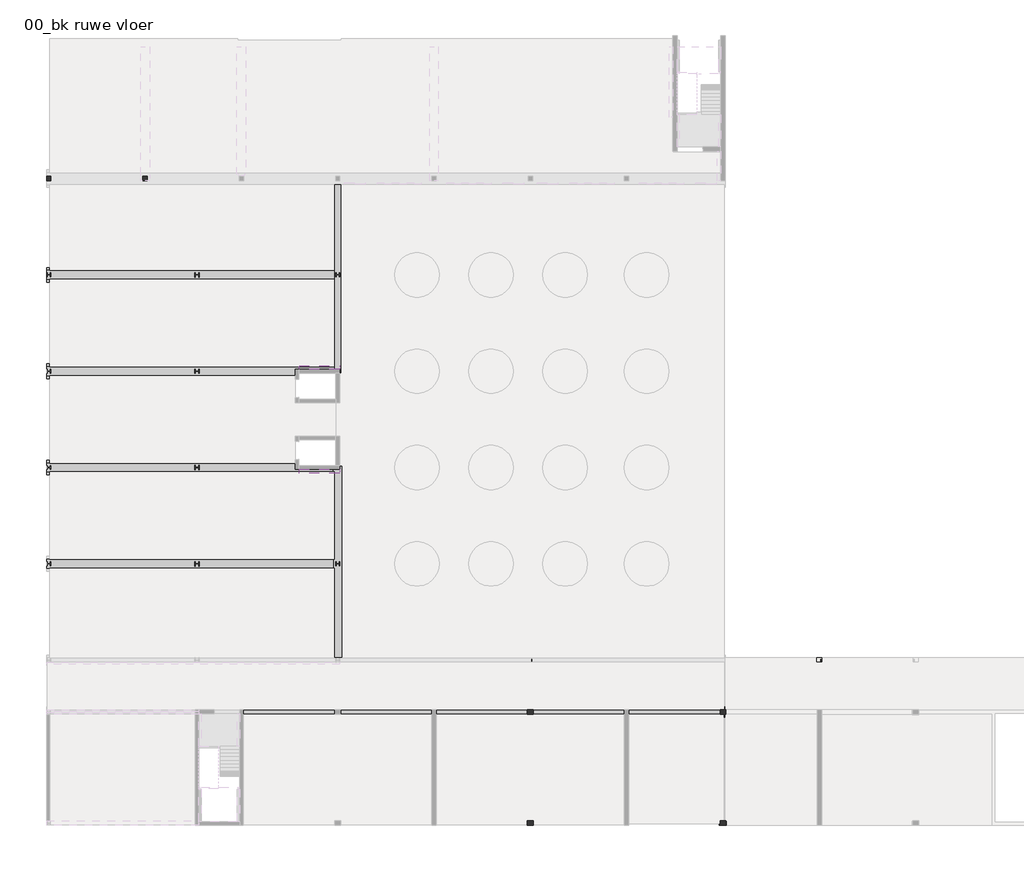
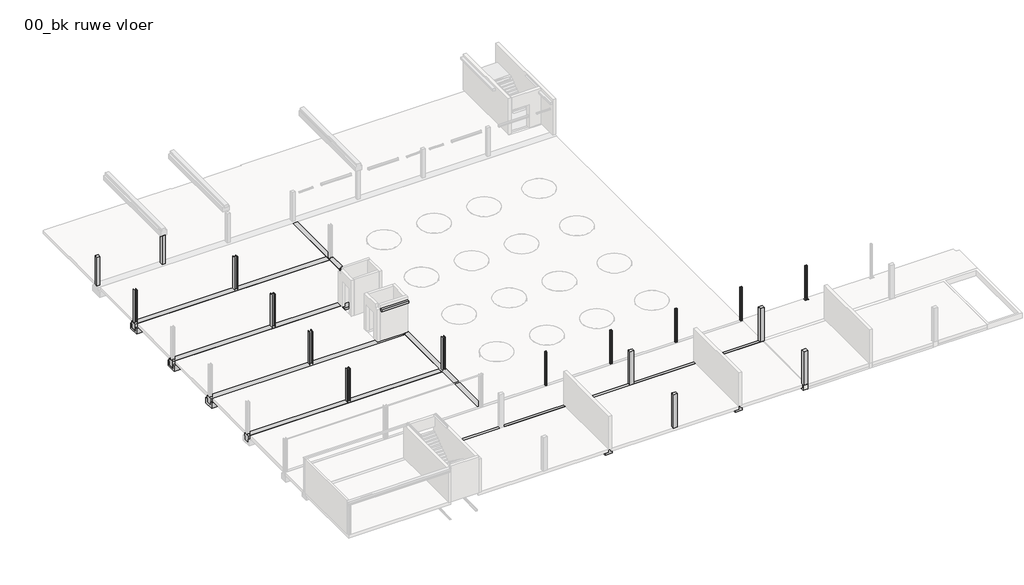
# One storey, part 5 of 6: 17 columns, 14 beams, 2 slabs.
# Revit data of these elements (continued)
# Type "NLRS_28_SF_LIB_balk dubbele sponning beton ihwg-CWV-MMBC-SRP_gen_rsf : balk beton ihwg_gen__bxh 900x900 met inkassing bxh 200x320" (continued)
#   RSF_C_breedte_inkassing_rechts = 200 mm
#   RSF_C_breedte_inkassing_links = 200 mm
#   NLRS_C_lengte [instance default] = 3000 mm
#   NLRS_C_hoogte = 900 mm
#   NLRS_C_breedte = 900 mm
#   Length [instance default] = 3000 mm
#   Structural Material = NLRS_f2_beton ihwg_gen_rsf
#   Model = ""
# Type "NLRS_22_SF_LIB_oplegnok beton prefab framing-CWV-MMBPC-SRP_gen_rsf : oplegnok beton prefab_gen__bxh 250x250/220"
#   Export Type to IFC As = "IfcWallType"
#   Type IfcGUID = "3EzArCxHzFqA2seU7O0xFZ"
#   Type Comments = "oplegnok"
#   Model = "LOD300"
#   Description = "oplegnok beton prefab 250x250/220"
#   Assembly Code = "22.11"
#   NLRS_C_hoogte_01 = 220 mm
#   NLRS_C_hoogte = 250 mm
#   NLRS_C_breedte = 250 mm
#   Lossing = 30 mm
#   Length [instance default] = 3000 mm
#   Structural Material = NLRS_f2_beton prefab_gen_rsf
# Type "NLRS_28_SCO_TLB_stalen kolom HEA-BCPG-MMBS-SRP_gen_rsf : stalen kolom_gen__HEA 260"
#   Type IFC Predefined Type = "COLUMN"
#   Export Type to IFC As = "IfcColumnType"
#   Type IfcGUID = "2$hNzCXOT3YR8V$0CfyzGd"
#   Type Comments = "HEA260"
#   Model = " "
#   Manufacturer = " "
#   Description = "stalen kolom HEA260"
#   Assembly Code = "28.11"
#   vz = 125 mm
#   vy = 130 mm
#   vpz = 125 mm
#   vpy = 130 mm
#   tw = 7.5 mm
#   tf = 12.5 mm
#   ra = 24 mm
#   d = 250 mm
#   bf = 260 mm
#   NLRS_C_lengte [instance default] = 2743.2 mm
#   Structural Material = NLRS_h2_staal_gen_rsf
#   Keynote = ""
# Type "NLRS_28_SCO_TLB_vierkante kolom beton prefab-BCPG-MMBPC-SRP_gen_rsf : kolom vierkant beton prefab_gen__bxh 300x300"
#   Type IFC Predefined Type = "COLUMN"
#   Export Type to IFC As = "IfcColumnType"
#   Type IfcGUID = "2bNskL0kfByRmbY5G6If0x"
#   Type Comments = "300x300"
#   Model = "LOD300"
#   Description = "prefab betonkolom 300x300"
#   Assembly Code = "28.11"
#   NLRS_C_lengte [instance default] = 2700 mm
#   NLRS_C_hoogte = 300 mm
#   NLRS_C_breedte = 300 mm
#   Structural Material = NLRS_f2_beton prefab_gen_rsf
# Type "NLRS_28_SCO_TLB_stalen kolom HEB-BCPG-MMBS-SRP_gen_rsf : stalen kolom_gen__HEB 300"
#   Type IFC Predefined Type = "COLUMN"
#   Export Type to IFC As = "IfcColumnType"
#   Type IfcGUID = "3C_b5Xdrv818Ti1jf59K4n"
#   Type Comments = "HEB300"
#   Model = " "
#   Manufacturer = " "
#   Description = "stalen kolom HEB300"
#   Assembly Code = "28.11"
#   vz = 150 mm
#   vy = 150 mm
#   vpz = 150 mm
#   vpy = 150 mm
#   tw = 11 mm
#   tf = 19 mm
#   ra = 27 mm
#   d = 300 mm
#   bf = 300 mm
#   NLRS_C_lengte [instance default] = 2743.2 mm
#   Structural Material = NLRS_h2_staal_gen_rsf
#   Keynote = ""
# Type "NLRS_28_SCO_TLB_vierkante kolom beton ihwg-BCPG-MMBC-SRP_gen_rsf : vierkante kolom beton ihwg_gen__bxh 400x300"
#   Type IFC Predefined Type = "COLUMN"
#   Export Type to IFC As = "IfcColumnType"
#   Type IfcGUID = "2lw04Qbvr9TgC3fLWwYn2N"
#   Type Comments = "400x300"
#   Model = "LOD300"
#   Description = "betonkolom ihwg 400x300"
#   Assembly Code = "28.11"
#   NLRS_C_lengte [instance default] = 2700 mm
#   NLRS_C_hoogte = 300 mm
#   NLRS_C_breedte = 400 mm
#   Structural Material = NLRS_f2_beton ihwg_gen_rsf
# Type "NLRS_28_SCO_TLB_stalen kolom buisprofiel koudgevormd vierkant-BCPG-MMBS-SRP_gen_rsf : stalen kolom buisprofiel koudgevormd vierkant RHSC_gen__160x160x8"
#   Type IFC Predefined Type = "COLUMN"
#   Export Type to IFC As = "IfcColumnType"
#   Type IfcGUID = "2$hNzCXOT3YR8V$0Cfyzxk"
#   Type Comments = "K160x160x8"
#   Model = " "
#   Manufacturer = " "
#   Description = "stalen kolom K160x160x8"
#   Assembly Code = "28.11"
#   vz = 80 mm
#   vy = 80 mm
#   vpz = 80 mm
#   vpy = 80 mm
#   tw = 8 mm
#   tf = 8 mm
#   ri = 20 mm
#   ra = 12 mm
#   d = 160 mm
#   bf = 160 mm
#   NLRS_C_lengte [instance default] = 2743.2 mm
#   Structural Material = NLRS_h2_staal_gen_rsf
#   Keynote = ""
# Type "NLRS_16_SFO_WPB_stiep rechthoek beton ihwg-AV-MMBC_gen_rsf : stiep beton ihwg_gen__bxl 300x400"
#   Export Type to IFC As = "IfcFootingType"
#   Type IfcGUID = "3aMdMHoe12P9KDGPyaIeli"
#   Type Comments = "stiep 300x400"
#   Description = "stiep 300x400"
#   Assembly Code = "16.13"
#   Width = 300 mm
#   NLRS_C_lengte = 400 mm
#   NLRS_C_hoogte [instance default] = 600 mm
#   NLRS_C_breedte = 300 mm
#   Length = 400 mm
#   Structural Material = NLRS_f2_beton ihwg_gen_rsf
#   Model = ""
#   Default Elevation = 0
# Type "NLRS_16_SFO_WPB_stiep rechthoek beton ihwg-AV-MMBC_gen_rsf : stiep beton ihwg_gen__bxl 300x500"
#   Export Type to IFC As = "IfcFootingType"
#   Type IfcGUID = "3aMdMHoe12P9KDGPyaIe1k"
#   Type Comments = "stiep 300x500"
#   Description = "stiep 300x500"
#   Assembly Code = "16.13"
#   Width = 300 mm
#   NLRS_C_lengte = 500 mm
#   NLRS_C_hoogte [instance default] = 600 mm
#   NLRS_C_breedte = 300 mm
#   Length = 500 mm
#   Structural Material = NLRS_f2_beton ihwg_gen_rsf
#   Model = ""
#   Default Elevation = 0
# Element 1 (IfcBeam, "NLRS_28_SF_LIB_balk dubbele sponning beton prefab-CWV-MMBC-SRP_gen_rsf : balk beton prefab_gen__bxh 700x700 met inkassing bxh 200x320")
#   IfcGUID = "0AFZSao6j3uApvehgmz3fE"
#   NLRS_C_lengte = 32650 mm
#   IsExternal = yes
#   LoadBearing = yes
#   Phase Created = NLRS_nieuw
#   Materials on its faces: "NLRS_f2_beton prefab_gen_rsf", "NLRS_f2_beton ihwg_gen_rsf"
# Element 2 (IfcBeam, "NLRS_28_SF_LIB_balk dubbele sponning beton ihwg-CWV-MMBC-SRP_gen_rsf : balk beton ihwg_gen__bxh 1000x900 met inkassing bxh 200x320")
#   IfcGUID = "2fqjgN40rEBBKvfwcj0B$q"
#   NLRS_C_lengte = 19900 mm
#   IsExternal = yes
#   LoadBearing = yes
#   Phase Created = NLRS_nieuw
#   Materials on its faces: "NLRS_f2_beton ihwg_gen_rsf"
# Element 3 (IfcBeam, "NLRS_28_SF_LIB_balk dubbele sponning beton ihwg-CWV-MMBC-SRP_gen_rsf : balk beton ihwg_gen__bxh 1000x900 met inkassing bxh 200x320")
#   IfcGUID = "2fqjgN40rEBBKvfwcj0Bzp"
#   NLRS_C_lengte = 19400 mm
#   IsExternal = yes
#   LoadBearing = yes
#   Phase Created = NLRS_nieuw
#   Materials on its faces: "NLRS_f2_beton ihwg_gen_rsf"
# Element 4 (IfcBeam, "NLRS_28_SF_LIB_balk dubbele sponning beton ihwg-CWV-MMBC-SRP_gen_rsf : balk beton ihwg_gen__bxh 1000x900 met inkassing bxh 200x320")
#   IfcGUID = "2fqjgN40rEBBKvfwcj0BzL"
#   NLRS_C_lengte = 19400 mm
#   IsExternal = yes
#   LoadBearing = yes
#   Phase Created = NLRS_nieuw
#   Materials on its faces: "NLRS_f2_beton ihwg_gen_rsf"
# Element 5 (IfcBeam, "NLRS_28_SF_LIB_balk dubbele sponning beton ihwg-CWV-MMBC-SRP_gen_rsf : balk beton ihwg_gen__bxh 1000x900 met inkassing bxh 200x320")
#   IfcGUID = "2fqjgN40rEBBKvfwcj0BY9"
#   NLRS_C_lengte = 19900 mm
#   IsExternal = yes
#   LoadBearing = yes
#   Phase Created = NLRS_nieuw
#   Materials on its faces: "NLRS_f2_beton ihwg_gen_rsf"
# Element 6 (IfcBeam, "NLRS_28_SF_LIB_balkbodem beton prefab-CWV-MMBC-SRP_gen_rsf : balkbodem beton prefab_gen__bxhxdk 1000x580x200")
#   IfcGUID = "0X0KViByb4JPBOa4XaNhJF"
#   NLRS_C_lengte = 19200 mm
#   IsExternal = yes
#   LoadBearing = yes
#   Phase Created = NLRS_nieuw
#   Materials on its faces: "NLRS_f2_beton prefab_gen_rsf"
# Element 7 (IfcBeam, "NLRS_28_SF_LIB_balkbodem beton prefab-CWV-MMBC-SRP_gen_rsf : balkbodem beton prefab_gen__bxhxdk 1000x580x200")
#   IfcGUID = "0X0KViByb4JPBOa4XaNgQF"
#   NLRS_C_lengte = 19200 mm
#   IsExternal = yes
#   LoadBearing = yes
#   Phase Created = NLRS_nieuw
#   Materials on its faces: "NLRS_f2_beton prefab_gen_rsf", "NLRS_f2_beton ihwg_gen_rsf"
# Element 8 (IfcBeam, "NLRS_28_SF_LIB_balkbodem beton prefab-CWV-MMBC-SRP_gen_rsf : balkbodem beton prefab_gen__bxhxdk 1000x580x200")
#   IfcGUID = "0X0KViByb4JPBOa4XaNgQc"
#   NLRS_C_lengte = 19200 mm
#   IsExternal = yes
#   LoadBearing = yes
#   Phase Created = NLRS_nieuw
#   Materials on its faces: "NLRS_f2_beton prefab_gen_rsf", "NLRS_f2_beton ihwg_gen_rsf"
# Element 9 (IfcBeam, "NLRS_28_SF_LIB_balk dubbele sponning beton ihwg-CWV-MMBC-SRP_gen_rsf : balk beton ihwg_gen__bxh 900x900 met inkassing bxh 200x320")
#   IfcGUID = "1E6t7WhRf97hJGfj3Bm3as"
#   NLRS_C_lengte = 12725 mm
#   IsExternal = yes
#   LoadBearing = yes
#   Phase Created = NLRS_nieuw
#   Materials on its faces: "NLRS_f2_beton ihwg_gen_rsf", "NLRS_f2_beton prefab_gen_rsf"
# Element 10 (IfcBeam, "NLRS_28_SF_LIB_balk dubbele sponning beton ihwg-CWV-MMBC-SRP_gen_rsf : balk beton ihwg_gen__bxh 1000x900 met inkassing bxh 200x320")
#   IfcGUID = "3iyfZByB98yevaQCZKiCcH"
#   NLRS_C_lengte = 12975 mm
#   IsExternal = yes
#   LoadBearing = yes
#   Phase Created = NLRS_nieuw
#   Materials on its faces: "NLRS_f2_beton ihwg_gen_rsf", "NLRS_f2_beton prefab_gen_rsf"
# Element 11 (IfcBeam, "NLRS_28_SF_LIB_balk dubbele sponning beton prefab-CWV-MMBC-SRP_gen_rsf : balk beton prefab_gen__bxh 700x700 met inkassing bxh 200x320")
#   IfcGUID = "3B2jA7IzvC4Aqddp_xdWat"
#   NLRS_C_lengte = 7500 mm
#   IsExternal = yes
#   LoadBearing = yes
#   Phase Created = NLRS_nieuw
#   Materials on its faces: "NLRS_f2_beton prefab_gen_rsf", "NLRS_f2_beton ihwg_gen_rsf"
# Element 12 (IfcBeam, "NLRS_28_SF_LIB_balk dubbele sponning beton prefab-CWV-MMBC-SRP_gen_rsf : balk beton prefab_gen__bxh 700x700 met inkassing bxh 200x320")
#   IfcGUID = "3B2jA7IzvC4Aqddp_xdWZ5"
#   NLRS_C_lengte = 7500 mm
#   IsExternal = yes
#   LoadBearing = yes
#   Phase Created = NLRS_nieuw
#   Materials on its faces: "NLRS_f2_beton prefab_gen_rsf", "NLRS_f2_beton ihwg_gen_rsf"
# Element 13 (IfcBeam, "NLRS_22_SF_LIB_oplegnok beton prefab framing-CWV-MMBPC-SRP_gen_rsf : oplegnok beton prefab_gen__bxh 250x250/220")
#   IfcGUID = "0zo1UjqZ91lRsfCKsOObF0"
#   IsExternal = no
#   LoadBearing = yes
#   Phase Created = NLRS_nieuw
#   Materials on its faces: "NLRS_f2_beton prefab_gen_rsf"
# Element 14 (IfcBeam, "NLRS_22_SF_LIB_oplegnok beton prefab framing-CWV-MMBPC-SRP_gen_rsf : oplegnok beton prefab_gen__bxh 250x250/220")
#   IfcGUID = "0zo1UjqZ91lRsfCKsOObqD"
#   IsExternal = no
#   LoadBearing = yes
#   Phase Created = NLRS_nieuw
#   Materials on its faces: "NLRS_f2_beton prefab_gen_rsf"
# Element 15 (IfcColumn, "NLRS_28_SCO_TLB_stalen kolom HEA-BCPG-MMBS-SRP_gen_rsf : stalen kolom_gen__HEA 260")
#   IfcGUID = "2$hNzCXOT3YR8V$0Cfyz1k"
#   Comments = ""
#   IsExternal = no
#   LoadBearing = yes
#   Phase Created = NLRS_nieuw
#   Materials on its faces: "NLRS_h2_staal_gen_rsf"
# Element 16 (IfcColumn, "NLRS_28_SCO_TLB_vierkante kolom beton prefab-BCPG-MMBPC-SRP_gen_rsf : kolom vierkant beton prefab_gen__bxh 300x300")
#   IfcGUID = "2$hNzCXOT3YR8V$0CfyzES"
#   IsExternal = no
#   LoadBearing = yes
#   Phase Created = NLRS_nieuw
#   Materials on its faces: "NLRS_f2_beton prefab_gen_rsf"
# Element 17 (IfcColumn, "NLRS_28_SCO_TLB_vierkante kolom beton prefab-BCPG-MMBPC-SRP_gen_rsf : kolom vierkant beton prefab_gen__bxh 300x300")
#   IfcGUID = "2ajLwCSRTE_9I1Spg4tpgS"
#   IsExternal = no
#   LoadBearing = yes
#   Phase Created = NLRS_nieuw
#   Materials on its faces: "NLRS_f2_beton prefab_gen_rsf"
# Element 18 (IfcColumn, "NLRS_28_SCO_TLB_stalen kolom HEB-BCPG-MMBS-SRP_gen_rsf : stalen kolom_gen__HEB 300")
#   IfcGUID = "2GRbcre991teoKeCLB8Lxx"
#   Comments = ""
#   IsExternal = no
#   LoadBearing = yes
#   Phase Created = NLRS_nieuw
#   Materials on its faces: "NLRS_h2_staal_gen_rsf"
# Element 19 (IfcColumn, "NLRS_28_SCO_TLB_stalen kolom HEB-BCPG-MMBS-SRP_gen_rsf : stalen kolom_gen__HEB 300")
#   IfcGUID = "2GRbcre991teoKeCLB8Lxv"
#   Comments = ""
#   IsExternal = no
#   LoadBearing = yes
#   Phase Created = NLRS_nieuw
#   Materials on its faces: "NLRS_h2_staal_gen_rsf"
# Element 20 (IfcColumn, "NLRS_28_SCO_TLB_stalen kolom HEB-BCPG-MMBS-SRP_gen_rsf : stalen kolom_gen__HEB 300")
#   IfcGUID = "2GRbcre991teoKeCLB8Lxd"
#   Comments = ""
#   IsExternal = no
#   LoadBearing = yes
#   Phase Created = NLRS_nieuw
#   Materials on its faces: "NLRS_h2_staal_gen_rsf"
# Element 21 (IfcColumn, "NLRS_28_SCO_TLB_stalen kolom HEB-BCPG-MMBS-SRP_gen_rsf : stalen kolom_gen__HEB 300")
#   IfcGUID = "2GRbcre991teoKeCLB8Lxb"
#   Comments = ""
#   IsExternal = no
#   LoadBearing = yes
#   Phase Created = NLRS_nieuw
#   Materials on its faces: "NLRS_h2_staal_gen_rsf"
# Element 22 (IfcColumn, "NLRS_28_SCO_TLB_stalen kolom HEA-BCPG-MMBS-SRP_gen_rsf : stalen kolom_gen__HEA 260")
#   IfcGUID = "2GRbcre991teoKeCLB8Lwq"
#   Comments = ""
#   IsExternal = no
#   LoadBearing = yes
#   Phase Created = NLRS_nieuw
#   Materials on its faces: "NLRS_h2_staal_gen_rsf"
# Element 23 (IfcColumn, "NLRS_28_SCO_TLB_vierkante kolom beton ihwg-BCPG-MMBC-SRP_gen_rsf : vierkante kolom beton ihwg_gen__bxh 400x300")
#   IfcGUID = "2lw04Qbvr9TgC3fLWwYn7K"
#   IsExternal = no
#   LoadBearing = yes
#   Phase Created = NLRS_nieuw
#   Materials on its faces: "NLRS_f2_beton ihwg_gen_rsf"
# Element 24 (IfcColumn, "NLRS_28_SCO_TLB_vierkante kolom beton ihwg-BCPG-MMBC-SRP_gen_rsf : vierkante kolom beton ihwg_gen__bxh 400x300")
#   IfcGUID = "2lw04Qbvr9TgC3fLWwYn61"
#   IsExternal = no
#   LoadBearing = yes
#   Phase Created = NLRS_nieuw
#   Materials on its faces: "NLRS_f2_beton ihwg_gen_rsf"
# Element 25 (IfcColumn, "NLRS_28_SCO_TLB_vierkante kolom beton ihwg-BCPG-MMBC-SRP_gen_rsf : vierkante kolom beton ihwg_gen__bxh 400x300")
#   IfcGUID = "2lw04Qbvr9TgC3fLWwYn5w"
#   IsExternal = no
#   LoadBearing = yes
#   Phase Created = NLRS_nieuw
#   Materials on its faces: "NLRS_f2_beton ihwg_gen_rsf"
# Element 26 (IfcColumn, "NLRS_28_SCO_TLB_vierkante kolom beton ihwg-BCPG-MMBC-SRP_gen_rsf : vierkante kolom beton ihwg_gen__bxh 400x300")
#   IfcGUID = "2lw04Qbvr9TgC3fLWwYn5T"
#   IsExternal = no
#   LoadBearing = yes
#   Phase Created = NLRS_nieuw
#   Materials on its faces: "NLRS_f2_beton ihwg_gen_rsf"
# Element 27 (IfcColumn, "NLRS_28_SCO_TLB_stalen kolom buisprofiel koudgevormd vierkant-BCPG-MMBS-SRP_gen_rsf : stalen kolom buisprofiel koudgevormd vierkant RHSC_gen__160x160x8")
#   IfcGUID = "2$hNzCXOT3YR8V$0Cfyzu5"
#   IsExternal = no
#   LoadBearing = yes
#   Phase Created = NLRS_nieuw
#   Materials on its faces: "NLRS_h2_staal_gen_rsf"
# Element 28 (IfcColumn, "NLRS_28_SCO_TLB_stalen kolom buisprofiel koudgevormd vierkant-BCPG-MMBS-SRP_gen_rsf : stalen kolom buisprofiel koudgevormd vierkant RHSC_gen__160x160x8")
#   IfcGUID = "2$hNzCXOT3YR8V$0Cfyzb1"
#   IsExternal = no
#   LoadBearing = yes
#   Phase Created = NLRS_nieuw
#   Materials on its faces: "NLRS_h2_staal_gen_rsf"
# Element 29 (IfcColumn, "NLRS_28_SCO_TLB_stalen kolom buisprofiel koudgevormd vierkant-BCPG-MMBS-SRP_gen_rsf : stalen kolom buisprofiel koudgevormd vierkant RHSC_gen__160x160x8")
#   IfcGUID = "2$hNzCXOT3YR8V$0CfyzZS"
#   IsExternal = no
#   LoadBearing = yes
#   Phase Created = NLRS_nieuw
#   Materials on its faces: "NLRS_h2_staal_gen_rsf"
# Element 30 (IfcColumn, "NLRS_28_SCO_TLB_stalen kolom buisprofiel koudgevormd vierkant-BCPG-MMBS-SRP_gen_rsf : stalen kolom buisprofiel koudgevormd vierkant RHSC_gen__160x160x8")
#   IfcGUID = "2$hNzCXOT3YR8V$0CfyzXQ"
#   IsExternal = no
#   LoadBearing = yes
#   Phase Created = NLRS_nieuw
#   Materials on its faces: "NLRS_h2_staal_gen_rsf"
# Element 31 (IfcColumn, "NLRS_28_SCO_TLB_stalen kolom buisprofiel koudgevormd vierkant-BCPG-MMBS-SRP_gen_rsf : stalen kolom buisprofiel koudgevormd vierkant RHSC_gen__160x160x8")
#   IfcGUID = "2$hNzCXOT3YR8V$0CfyzlM"
#   IsExternal = no
#   LoadBearing = yes
#   Phase Created = NLRS_nieuw
#   Materials on its faces: "NLRS_h2_staal_gen_rsf"
# Element 32 (IfcSlab, "NLRS_16_SFO_WPB_stiep rechthoek beton ihwg-AV-MMBC_gen_rsf : stiep beton ihwg_gen__bxl 300x400")
#   IfcGUID = "3aMdMHoe12P9KDGPyaIelA"
#   NLRS_C_hoogte = 520 mm
#   IsExternal = yes
#   LoadBearing = yes
#   Phase Created = NLRS_nieuw
#   Materials on its faces: "NLRS_f2_beton ihwg_gen_rsf"
# Element 33 (IfcSlab, "NLRS_16_SFO_WPB_stiep rechthoek beton ihwg-AV-MMBC_gen_rsf : stiep beton ihwg_gen__bxl 300x500")
#   IfcGUID = "2LiCovvSXDMQbhYz9hLID3"
#   NLRS_C_hoogte = 520 mm
#   IsExternal = yes
#   LoadBearing = yes
#   Phase Created = NLRS_nieuw
#   Materials on its faces: "NLRS_f2_beton ihwg_gen_rsf"
# Materials
#   "NLRS_f2_beton prefab_gen_rsf": class "F - Niet gebakken kunststeen", colour RGB 129 133 118, transparency 0, Keynote = "f2", Manufacturer = "Revit Standards Foundation", URL = "www.revitstandards.org", Description = "beton prefab", Cost = 0
#   "NLRS_f2_beton ihwg_gen_rsf": class "F - Niet gebakken kunststeen", colour RGB 129 133 118, transparency 0, Keynote = "f2", Manufacturer = "Revit Standards Foundation", URL = "www.revitstandards.org", Description = "beton ihwg", Cost = 0
#   "NLRS_h2_staal_gen_rsf": class "H - Metaal", colour RGB 189 187 185, transparency 0, Keynote = "h2", Manufacturer = "Revit Standards Foundation", URL = "www.revitstandards.org", Description = "staal", Cost = 0
# Room, not placed, phase "NLRS_bestaand", upper offset 0 mm, lower offset 0 mm
#   Number = "1"
#   Name = "Room"
